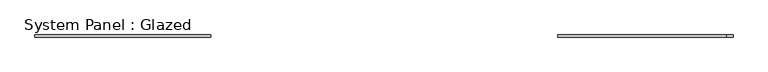
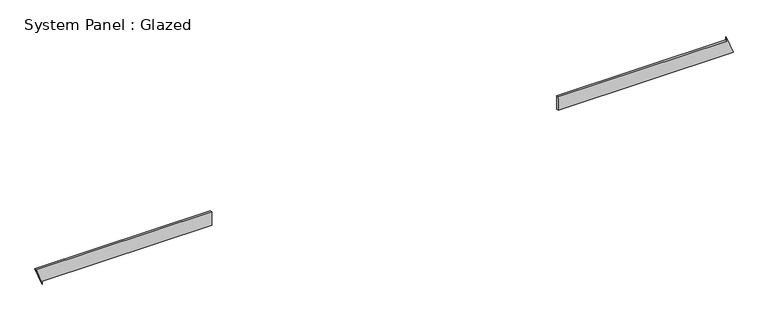
"""IFC4 building model written with IfcOpenShell, lengths in millimetres: plate geometry, System Panel : Glazed."""

from ifc_helpers import new_model, si_unit, frame, origin, place, context, project, spatial, polyline, outline, extrude, source, transform, mapped, element, save


def system_panel_glazed_01b56bff(model_context):
    return source(origin(), model_context, "Body", "SweptSolid", [
        extrude(outline(polyline([(0.0, -3956.991033), (35.3553391, -3956.991033), (35.3553391, -1998.813369), (198.561189, -2000.3469562), (198.6124026, -4027.528574), (0.0, -3956.991033)])), frame((0.0, -49.5, 0.0), z_axis=(0.0, 1.0, 0.0), x_axis=(0.0, 0.0, 1.0)), (0.0, 0.0, 1.0), 25.0),
        extrude(outline(polyline([(35.3553391, 2005.1688647), (35.3553391, 4027.528574), (233.766037, 3956.5208191), (198.410698, 3956.5199259), (198.4599572, 2006.6977747), (35.3553391, 2005.1688647)])), frame((0.0, -49.5, 0.0), z_axis=(0.0, 1.0, 0.0), x_axis=(0.0, 0.0, 1.0)), (0.0, 0.0, 1.0), 25.0),
    ])


if __name__ == "__main__":
    model = new_model("IFC4")
    model_context = context("Model", 3, world=origin())
    ifc_project = project(units=[si_unit("LENGTHUNIT", "METRE", prefix="MILLI")], contexts=[model_context])
    site = spatial("IfcSite", under=ifc_project)
    building = spatial("IfcBuilding", under=site)
    placement = place(None, origin())
    system_panel_glazed_shape = system_panel_glazed_01b56bff(model_context)
    element("IfcPlate", 1, ObjectType="System Panel : Glazed", at=placement, inside=building, context=model_context, shape_type="MappedRepresentation", body=[
        mapped(system_panel_glazed_shape, transform((0.0, 0.0, 0.0), x_axis=(1.0, 0.0, 0.0), y_axis=(0.0, 1.0, 0.0), z_axis=(0.0, 0.0, 1.0))),
    ])
    save(model, "model.ifc")

# Revit data of these elements
# Element 1 (IfcPlate, "System Panel : Glazed")
#   Materials on its faces: "Glass"
# Materials
#   "Glass": class "Glass", colour RGB 218 227 224, transparency 0.85, Description = "Soda Lime Glass", Cost = 0
